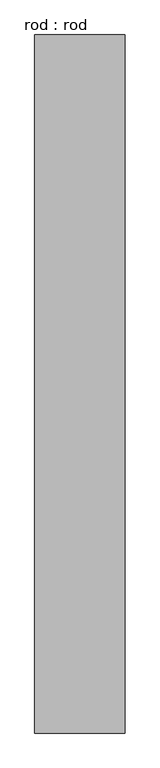
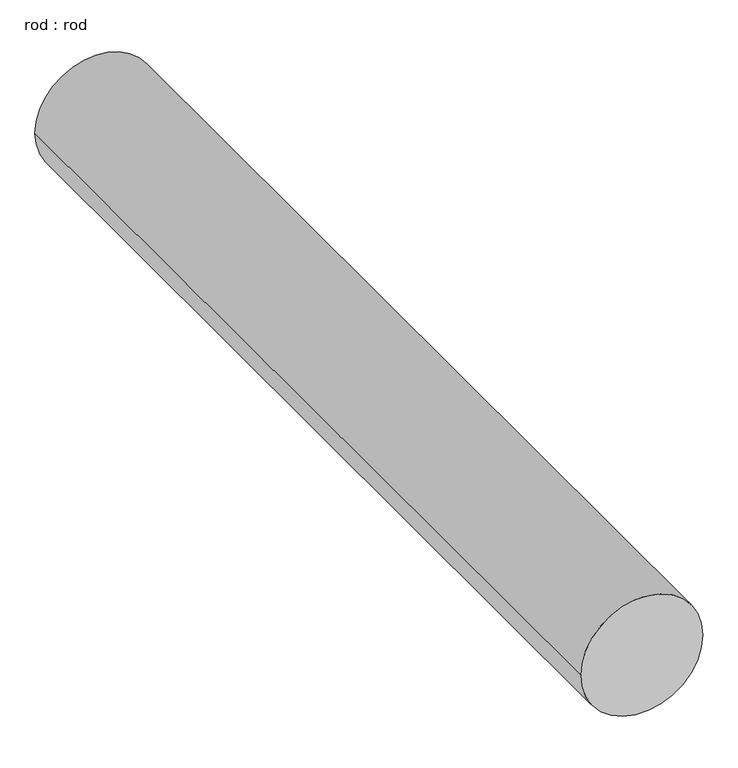
"""IFC4 building model written with IfcOpenShell, lengths in millimetres: proxy geometry, rod : rod."""

from ifc_helpers import new_model, si_unit, point, frame, frame_2d, origin, place, context, project, spatial, circle_curve, trimmed, segment, composite_curve, outline, extrude, source, transform, mapped, element, save


def rod_rod_5086bad4(model_context):
    return source(origin(), model_context, "Body", "SweptSolid", [
        extrude(outline(composite_curve([segment(trimmed(circle_curve(frame_2d((0.0108462, 0.0)), 200.0), [point((0.0108462, 200.0))], [point((0.0108462, -200.0))], False, "CARTESIAN"), True, "CONTINUOUS"), segment(trimmed(circle_curve(frame_2d((0.0108462, 0.0)), 200.0), [point((0.0108462, -200.0))], [point((0.0108462, 200.0))], False, "CARTESIAN"), True, "CONTINUOUS")], self_intersect=False)), frame((0.0, 2544.5143296, 0.0), z_axis=(0.0, 1.0, 0.0), x_axis=(0.0, 0.0, 1.0)), (0.0, 0.0, 1.0), 3096.4285714),
    ])


if __name__ == "__main__":
    model = new_model("IFC4")
    model_context = context("Model", 3, world=origin())
    ifc_project = project(units=[si_unit("LENGTHUNIT", "METRE", prefix="MILLI")], contexts=[model_context])
    site = spatial("IfcSite", under=ifc_project)
    building = spatial("IfcBuilding", under=site)
    placement = place(None, origin())
    rod_rod_shape = rod_rod_5086bad4(model_context)
    element("IfcBuildingElementProxy", 1, Name="rod : rod", ObjectType="rod : rod", at=placement, inside=building, context=model_context, shape_type="MappedRepresentation", body=[
        mapped(rod_rod_shape, transform((0.0, 0.0, 0.0), x_axis=(1.0, 0.0, 0.0), y_axis=(0.0, 1.0, 0.0), z_axis=(0.0, 0.0, 1.0))),
    ])
    save(model, "model.ifc")

# Revit data of these elements
# Type "rod : rod"
#   Default Elevation = 0
